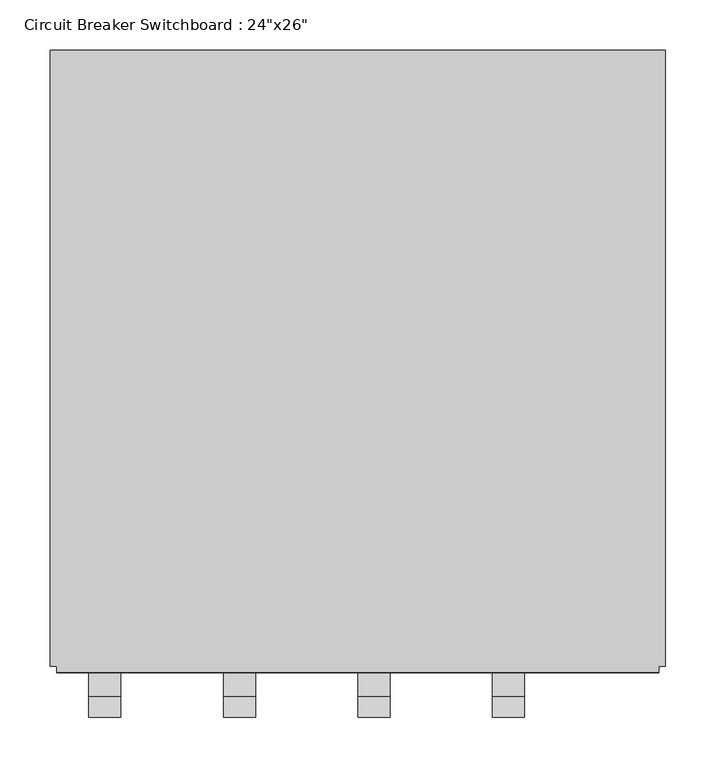
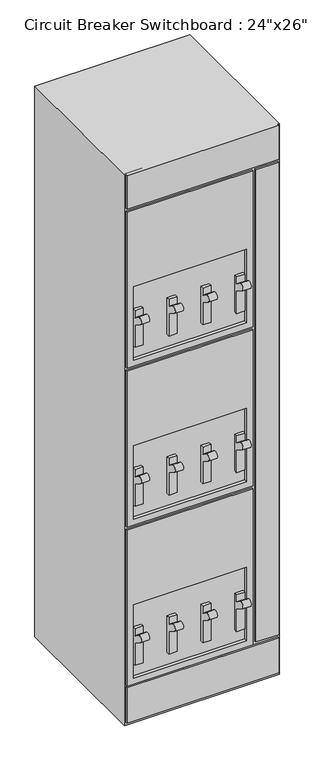
"""IFC4 building model written with IfcOpenShell, lengths in millimetres: proxy geometry."""

from ifc_helpers import new_model, si_unit, point, frame, frame_2d, origin, origin_with_axes, place, context, project, spatial, polyline, circle_curve, trimmed, segment, composite_curve, outline, extrude, faceted_brep, source, transform, mapped, element, save


def proxy_5f9e3781(model_context):
    return source(origin(), model_context, "Body", "SolidModel", [
        extrude(outline(composite_curve([segment(polyline([(-639.9115662, 381.1284675), (-616.1854499, 365.125), (-616.1854499, 393.7), (-603.4854499, 393.7), (-603.4854499, 241.3), (-616.1854499, 241.3), (-616.1854499, 333.375), (-654.6306098, 359.3065878)]), True, "CONTINUOUS"), segment(trimmed(circle_curve(frame_2d((-647.271088, 370.2175277)), 13.1609715), [point((-654.6306098, 359.3065878))], [point((-639.9115662, 381.1284675))], False, "CARTESIAN"), True, "CONTINUOUS")], self_intersect=False)), frame((133.35, 0.0, 0.0), z_axis=(1.0, 0.0, 0.0), x_axis=(0.0, 1.0, 0.0)), (0.0, 0.0, 1.0), 31.75),
        extrude(outline(composite_curve([segment(polyline([(-639.9115662, 381.1284675), (-616.1854499, 365.125), (-616.1854499, 393.7), (-603.4854499, 393.7), (-603.4854499, 241.3), (-616.1854499, 241.3), (-616.1854499, 333.375), (-654.6306098, 359.3065878)]), True, "CONTINUOUS"), segment(trimmed(circle_curve(frame_2d((-647.271088, 370.2175277)), 13.1609715), [point((-654.6306098, 359.3065878))], [point((-639.9115662, 381.1284675))], False, "CARTESIAN"), True, "CONTINUOUS")], self_intersect=False)), frame((0.0, 0.0, 0.0), z_axis=(1.0, 0.0, 0.0), x_axis=(0.0, 1.0, 0.0)), (0.0, 0.0, 1.0), 31.75),
        extrude(outline(composite_curve([segment(polyline([(-639.9115662, 381.1284675), (-616.1854499, 365.125), (-616.1854499, 393.7), (-603.4854499, 393.7), (-603.4854499, 241.3), (-616.1854499, 241.3), (-616.1854499, 333.375), (-654.6306098, 359.3065878)]), True, "CONTINUOUS"), segment(trimmed(circle_curve(frame_2d((-647.271088, 370.2175277)), 13.1609715), [point((-654.6306098, 359.3065878))], [point((-639.9115662, 381.1284675))], False, "CARTESIAN"), True, "CONTINUOUS")], self_intersect=False)), frame((-133.35, 0.0, 0.0), z_axis=(1.0, 0.0, 0.0), x_axis=(0.0, 1.0, 0.0)), (0.0, 0.0, 1.0), 31.75),
        extrude(outline(composite_curve([segment(polyline([(-639.9115662, 381.1284675), (-616.1854499, 365.125), (-616.1854499, 393.7), (-603.4854499, 393.7), (-603.4854499, 241.3), (-616.1854499, 241.3), (-616.1854499, 333.375), (-654.6306098, 359.3065878)]), True, "CONTINUOUS"), segment(trimmed(circle_curve(frame_2d((-647.271088, 370.2175277)), 13.1609715), [point((-654.6306098, 359.3065878))], [point((-639.9115662, 381.1284675))], False, "CARTESIAN"), True, "CONTINUOUS")], self_intersect=False)), frame((-266.7, 0.0, 0.0), z_axis=(1.0, 0.0, 0.0), x_axis=(0.0, 1.0, 0.0)), (0.0, 0.0, 1.0), 31.75),
        extrude(outline(composite_curve([segment(polyline([(-639.9115662, 1041.5284675), (-616.1854499, 1025.525), (-616.1854499, 1054.1), (-603.4854499, 1054.1), (-603.4854499, 901.7), (-616.1854499, 901.7), (-616.1854499, 993.775), (-654.6306098, 1019.7065878)]), True, "CONTINUOUS"), segment(trimmed(circle_curve(frame_2d((-647.271088, 1030.6175277)), 13.1609715), [point((-654.6306098, 1019.7065878))], [point((-639.9115662, 1041.5284675))], False, "CARTESIAN"), True, "CONTINUOUS")], self_intersect=False)), frame((133.35, 0.0, 0.0), z_axis=(1.0, 0.0, 0.0), x_axis=(0.0, 1.0, 0.0)), (0.0, 0.0, 1.0), 31.75),
        extrude(outline(composite_curve([segment(polyline([(-639.9115662, 1041.5284675), (-616.1854499, 1025.525), (-616.1854499, 1054.1), (-603.4854499, 1054.1), (-603.4854499, 901.7), (-616.1854499, 901.7), (-616.1854499, 993.775), (-654.6306098, 1019.7065878)]), True, "CONTINUOUS"), segment(trimmed(circle_curve(frame_2d((-647.271088, 1030.6175277)), 13.1609715), [point((-654.6306098, 1019.7065878))], [point((-639.9115662, 1041.5284675))], False, "CARTESIAN"), True, "CONTINUOUS")], self_intersect=False)), frame((0.0, 0.0, 0.0), z_axis=(1.0, 0.0, 0.0), x_axis=(0.0, 1.0, 0.0)), (0.0, 0.0, 1.0), 31.75),
        extrude(outline(composite_curve([segment(polyline([(-639.9115662, 1041.5284675), (-616.1854499, 1025.525), (-616.1854499, 1054.1), (-603.4854499, 1054.1), (-603.4854499, 901.7), (-616.1854499, 901.7), (-616.1854499, 993.775), (-654.6306098, 1019.7065878)]), True, "CONTINUOUS"), segment(trimmed(circle_curve(frame_2d((-647.271088, 1030.6175277)), 13.1609715), [point((-654.6306098, 1019.7065878))], [point((-639.9115662, 1041.5284675))], False, "CARTESIAN"), True, "CONTINUOUS")], self_intersect=False)), frame((-133.35, 0.0, 0.0), z_axis=(1.0, 0.0, 0.0), x_axis=(0.0, 1.0, 0.0)), (0.0, 0.0, 1.0), 31.75),
        extrude(outline(composite_curve([segment(polyline([(-639.9115662, 1041.5284675), (-616.1854499, 1025.525), (-616.1854499, 1054.1), (-603.4854499, 1054.1), (-603.4854499, 901.7), (-616.1854499, 901.7), (-616.1854499, 993.775), (-654.6306098, 1019.7065878)]), True, "CONTINUOUS"), segment(trimmed(circle_curve(frame_2d((-647.271088, 1030.6175277)), 13.1609715), [point((-654.6306098, 1019.7065878))], [point((-639.9115662, 1041.5284675))], False, "CARTESIAN"), True, "CONTINUOUS")], self_intersect=False)), frame((-266.7, 0.0, 0.0), z_axis=(1.0, 0.0, 0.0), x_axis=(0.0, 1.0, 0.0)), (0.0, 0.0, 1.0), 31.75),
        extrude(outline(composite_curve([segment(polyline([(-639.9115662, 1701.9284675), (-616.1854499, 1685.925), (-616.1854499, 1714.5), (-603.4854499, 1714.5), (-603.4854499, 1562.1), (-616.1854499, 1562.1), (-616.1854499, 1654.175), (-654.6306098, 1680.1065878)]), True, "CONTINUOUS"), segment(trimmed(circle_curve(frame_2d((-647.271088, 1691.0175277)), 13.1609715), [point((-654.6306098, 1680.1065878))], [point((-639.9115662, 1701.9284675))], False, "CARTESIAN"), True, "CONTINUOUS")], self_intersect=False)), frame((133.35, 0.0, 0.0), z_axis=(1.0, 0.0, 0.0), x_axis=(0.0, 1.0, 0.0)), (0.0, 0.0, 1.0), 31.75),
        extrude(outline(composite_curve([segment(polyline([(-639.9115662, 1701.9284675), (-616.1854499, 1685.925), (-616.1854499, 1714.5), (-603.4854499, 1714.5), (-603.4854499, 1562.1), (-616.1854499, 1562.1), (-616.1854499, 1654.175), (-654.6306098, 1680.1065878)]), True, "CONTINUOUS"), segment(trimmed(circle_curve(frame_2d((-647.271088, 1691.0175277)), 13.1609715), [point((-654.6306098, 1680.1065878))], [point((-639.9115662, 1701.9284675))], False, "CARTESIAN"), True, "CONTINUOUS")], self_intersect=False)), frame((0.0, 0.0, 0.0), z_axis=(1.0, 0.0, 0.0), x_axis=(0.0, 1.0, 0.0)), (0.0, 0.0, 1.0), 31.75),
        extrude(outline(composite_curve([segment(polyline([(-639.9115662, 1701.9284675), (-616.1854499, 1685.925), (-616.1854499, 1714.5), (-603.4854499, 1714.5), (-603.4854499, 1562.1), (-616.1854499, 1562.1), (-616.1854499, 1654.175), (-654.6306098, 1680.1065878)]), True, "CONTINUOUS"), segment(trimmed(circle_curve(frame_2d((-647.271088, 1691.0175277)), 13.1609715), [point((-654.6306098, 1680.1065878))], [point((-639.9115662, 1701.9284675))], False, "CARTESIAN"), True, "CONTINUOUS")], self_intersect=False)), frame((-133.35, 0.0, 0.0), z_axis=(1.0, 0.0, 0.0), x_axis=(0.0, 1.0, 0.0)), (0.0, 0.0, 1.0), 31.75),
        extrude(outline(composite_curve([segment(polyline([(-639.9115662, 1701.9284675), (-616.1854499, 1685.925), (-616.1854499, 1714.5), (-603.4854499, 1714.5), (-603.4854499, 1562.1), (-616.1854499, 1562.1), (-616.1854499, 1654.175), (-654.6306098, 1680.1065878)]), True, "CONTINUOUS"), segment(trimmed(circle_curve(frame_2d((-647.271088, 1691.0175277)), 13.1609715), [point((-654.6306098, 1680.1065878))], [point((-639.9115662, 1701.9284675))], False, "CARTESIAN"), True, "CONTINUOUS")], self_intersect=False)), frame((-266.7, 0.0, 0.0), z_axis=(1.0, 0.0, 0.0), x_axis=(0.0, 1.0, 0.0)), (0.0, 0.0, 1.0), 31.75),
        faceted_brep([(-304.8, -609.8354499, 2286.0), (-304.8, -609.8354499, 0.0), (304.8, -609.8354499, 0.0), (304.8, -609.8354499, 2286.0), (298.45, -609.8354499, 2286.0), (298.45, -609.8354499, 2146.3), (-298.45, -609.8354499, 2146.3), (-298.45, -609.8354499, 2286.0), (-298.45, -609.8354499, 812.8), (196.85, -609.8354499, 812.8), (196.85, -609.8354499, 165.1), (-298.45, -609.8354499, 165.1), (-298.45, -609.8354499, 1473.2), (196.85, -609.8354499, 1473.2), (196.85, -609.8354499, 825.5), (-298.45, -609.8354499, 825.5), (-298.45, -609.8354499, 2133.6), (196.85, -609.8354499, 2133.6), (196.85, -609.8354499, 1485.9), (-298.45, -609.8354499, 1485.9), (209.55, -609.8354499, 2133.6), (298.45, -609.8354499, 2133.6), (298.45, -609.8354499, 171.45), (209.55, -609.8354499, 171.45), (-298.45, -609.8354499, 158.75), (298.45, -609.8354499, 158.75), (298.45, -609.8354499, 12.7), (-298.45, -609.8354499, 12.7), (304.8, 0.0, 2286.0), (304.8, 0.0, 0.0), (-304.8, 0.0, 0.0), (-304.8, 0.0, 2286.0), (-298.45, -616.1854499, 2286.0), (298.45, -616.1854499, 2286.0), (171.45, -603.4854499, 1816.1), (-273.05, -603.4854499, 1816.1), (-273.05, -603.4854499, 1511.3), (171.45, -603.4854499, 1511.3), (171.45, -616.1854499, 1816.1), (-273.05, -616.1854499, 1816.1), (-273.05, -616.1854499, 1511.3), (171.45, -616.1854499, 1511.3), (171.45, -603.4854499, 1155.7), (-273.05, -603.4854499, 1155.7), (-273.05, -603.4854499, 850.9), (171.45, -603.4854499, 850.9), (171.45, -616.1854499, 1155.7), (-273.05, -616.1854499, 1155.7), (-273.05, -616.1854499, 850.9), (171.45, -616.1854499, 850.9), (196.85, -616.1854499, 812.8), (-298.45, -616.1854499, 812.8), (-298.45, -616.1854499, 165.1), (196.85, -616.1854499, 165.1), (-273.05, -616.1854499, 495.3), (171.45, -616.1854499, 495.3), (171.45, -616.1854499, 190.5), (-273.05, -616.1854499, 190.5), (171.45, -603.4854499, 495.3), (-273.05, -603.4854499, 495.3), (-273.05, -603.4854499, 190.5), (171.45, -603.4854499, 190.5), (196.85, -616.1854499, 1473.2), (-298.45, -616.1854499, 1473.2), (-298.45, -616.1854499, 825.5), (196.85, -616.1854499, 825.5), (196.85, -616.1854499, 2133.6), (-298.45, -616.1854499, 2133.6), (-298.45, -616.1854499, 1485.9), (196.85, -616.1854499, 1485.9), (-298.45, -616.1854499, 2146.3), (298.45, -616.1854499, 2146.3), (298.45, -616.1854499, 2133.6), (209.55, -616.1854499, 2133.6), (209.55, -616.1854499, 171.45), (298.45, -616.1854499, 171.45), (298.45, -616.1854499, 158.75), (-298.45, -616.1854499, 158.75), (-298.45, -616.1854499, 12.7), (298.45, -616.1854499, 12.7)], [[[0, 1, 2, 3, 4, 5, 6, 7], [8, 9, 10, 11], [12, 13, 14, 15], [16, 17, 18, 19], [20, 21, 22, 23], [24, 25, 26, 27]], [[28, 29, 30, 31]], [[28, 31, 0, 7, 32, 33, 4, 3]], [[1, 0, 31, 30]], [[2, 1, 30, 29]], [[3, 2, 29, 28]], [[34, 35, 36, 37]], [[35, 34, 38, 39]], [[36, 35, 39, 40]], [[37, 36, 40, 41]], [[34, 37, 41, 38]], [[42, 43, 44, 45]], [[43, 42, 46, 47]], [[44, 43, 47, 48]], [[45, 44, 48, 49]], [[42, 45, 49, 46]], [[50, 51, 52, 53], [54, 55, 56, 57]], [[51, 50, 9, 8]], [[52, 51, 8, 11]], [[53, 52, 11, 10]], [[50, 53, 10, 9]], [[58, 59, 60, 61]], [[59, 58, 55, 54]], [[60, 59, 54, 57]], [[61, 60, 57, 56]], [[58, 61, 56, 55]], [[62, 63, 64, 65], [47, 46, 49, 48]], [[63, 62, 13, 12]], [[64, 63, 12, 15]], [[65, 64, 15, 14]], [[62, 65, 14, 13]], [[66, 67, 68, 69], [39, 38, 41, 40]], [[67, 66, 17, 16]], [[68, 67, 16, 19]], [[69, 68, 19, 18]], [[66, 69, 18, 17]], [[33, 32, 70, 71]], [[70, 32, 7, 6]], [[71, 70, 6, 5]], [[33, 71, 5, 4]], [[72, 73, 74, 75]], [[73, 72, 21, 20]], [[74, 73, 20, 23]], [[75, 74, 23, 22]], [[72, 75, 22, 21]], [[76, 77, 78, 79]], [[77, 76, 25, 24]], [[78, 77, 24, 27]], [[79, 78, 27, 26]], [[76, 79, 26, 25]]]),
        extrude(outline(polyline([(304.8, 0.0), (304.8, -603.4854499), (-304.8, -603.4854499), (-304.8, 0.0), (304.8, 0.0)])), origin_with_axes(), (0.0, 0.0, 1.0), 2286.0),
    ])


if __name__ == "__main__":
    model = new_model("IFC4")
    model_context = context("Model", 3, world=origin())
    ifc_project = project(units=[si_unit("LENGTHUNIT", "METRE", prefix="MILLI")], contexts=[model_context])
    site = spatial("IfcSite", under=ifc_project)
    building = spatial("IfcBuilding", under=site)
    placement = place(None, origin())
    proxy_shape = proxy_5f9e3781(model_context)
    element("IfcBuildingElementProxy", 1, Name="Circuit Breaker Switchboard : 24\"x26\"", ObjectType="Circuit Breaker Switchboard : 24\"x26\"", at=placement, inside=building, context=model_context, shape_type="MappedRepresentation", body=[
        mapped(proxy_shape, transform((0.0, 0.0, 0.0), x_axis=(1.0, 0.0, 0.0), y_axis=(0.0, 1.0, 0.0), z_axis=(0.0, 0.0, 1.0))),
    ])
    save(model, "model.ifc")

# Revit data of these elements
# Type "Circuit Breaker Switchboard : 24\"x26\""
#   Switchboard Width = 2' - 2"
#   Switchboard Voltage = 480 V
#   Switchboard Length = 2' - 0"
#   Switchboard Height = 7' - 6"
#   Length = 0' - 0 1/4"
#   Switch Visibility = yes
#   Switch Count = 4
#   Number of Poles = 3
#   Switchboard Material = none
#   Switch Material = none
